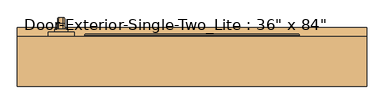
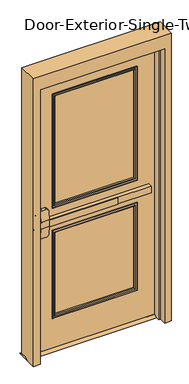
"""IFC4 building model written with IfcOpenShell, lengths in millimetres: door geometry."""

from ifc_helpers import new_model, si_unit, point, frame, frame_2d, origin, place, context, project, spatial, polyline, circle_curve, ellipse_curve, trimmed, segment, composite_curve, outline, extrude, faceted_brep, source, transform, mapped, element, save
from ifc_brep_helpers import plane_surface, cylinder_surface, revolved_surface, advanced_brep


def door_7385851d(model_context):
    return source(origin(), model_context, "Body", "SolidModel", [
        extrude(outline(polyline([(12.7, 12.7), (57.15, 12.7), (82.55, 0.0), (-12.7, 0.0), (12.7, 12.7)])), frame((-508.0, 0.0, 0.0), z_axis=(1.0, 0.0, 0.0), x_axis=(0.0, 1.0, 0.0)), (0.0, 0.0, 1.0), 1016.0),
        extrude(outline(polyline([(150.2833333, -25.4), (-349.25, -25.4), (-349.25, -19.05), (150.2833333, -19.05), (150.2833333, -25.4)])), frame((0.0, 0.0, 990.6), z_axis=(0.0, 0.0, 1.0), x_axis=(1.0, 0.0, 0.0)), (0.0, 0.0, 1.0), 50.8),
        advanced_brep(
        [(-412.75, -19.05, 1041.4), (-412.75, -19.05, 990.6), (-349.25, -19.05, 990.6), (400.05, -19.05, 990.6), (400.05, -19.05, 1041.4), (-349.25, -19.05, 1041.4), (400.05, 12.7, 1041.4), (400.05, 12.7, 990.6), (-349.25, 12.7, 990.6), (-349.25, 12.7, 927.1), (-368.3, 12.7, 908.05), (-393.7, 12.7, 908.05), (-412.75, 12.7, 927.1), (-412.75, 12.7, 1104.9), (-393.7, 12.7, 1123.95), (-368.3, 12.7, 1123.95), (-349.25, 12.7, 1104.9), (-349.25, 12.7, 1041.4), (-349.25, -15.8747533, 1041.4), (-412.75, -15.8747533, 1041.4), (-412.75, -10.8645731, 1104.9), (-412.75, -10.8645731, 927.1), (-412.75, -15.8747533, 990.6), (-349.25, -15.8747533, 990.6), (-349.25, -10.8645731, 927.1), (-349.25, -10.8645731, 1104.9), (-393.7, -9.361519, 1123.95), (-368.3, -9.361519, 1123.95), (-368.3, -9.361519, 908.05), (-393.7, -9.361519, 908.05)],
        [
            (0, 1),
            (1, 2),
            (2, 3),
            (3, 4),
            (4, 5),
            (5, 0),
            (6, 7),
            (7, 8),
            (8, 9),
            (9, 10, circle_curve(frame((-368.3, 12.7, 927.1), z_axis=(0.0, 1.0, 0.0), x_axis=(1.0, 0.0, 0.0)), 19.05)),
            (10, 11),
            (11, 12, circle_curve(frame((-393.7, 12.7, 927.1), z_axis=(0.0, 1.0, 0.0), x_axis=(1.0, 0.0, 0.0)), 19.05)),
            (12, 13),
            (13, 14, circle_curve(frame((-393.7, 12.7, 1104.9), z_axis=(0.0, 1.0, 0.0), x_axis=(1.0, 0.0, 0.0)), 19.05)),
            (14, 15),
            (15, 16, circle_curve(frame((-368.3, 12.7, 1104.9), z_axis=(0.0, 1.0, 0.0), x_axis=(1.0, 0.0, 0.0)), 19.05)),
            (16, 17),
            (17, 6),
            (4, 6),
            (17, 18),
            (18, 19),
            (19, 0),
            (19, 20),
            (20, 13),
            (12, 21),
            (21, 22),
            (22, 1),
            (7, 3),
            (22, 23),
            (23, 8),
            (23, 24),
            (24, 9),
            (16, 25),
            (25, 18),
            (14, 26),
            (26, 27),
            (27, 15),
            (10, 28),
            (28, 29),
            (29, 11),
            (24, 28, ellipse_curve(frame((-368.3, -10.8645731, 927.1), z_axis=(0.0, 0.9969018152893365, 0.07865602756830282), x_axis=(0.0, -0.07865602756830208, 0.9969018152893365)), 19.1092038, 19.05)),
            (27, 25, ellipse_curve(frame((-368.3, -10.8645731, 1104.9), z_axis=(0.0, 0.9969018152893376, -0.07865602756828934), x_axis=(0.0, -0.078656027568288, -0.9969018152893377)), 19.1092038, 19.05)),
            (20, 26, ellipse_curve(frame((-393.7, -10.8645731, 1104.9), z_axis=(0.0, 0.9969018152893376, -0.07865602756828934), x_axis=(0.0, -0.078656027568288, -0.9969018152893377)), 19.1092038, 19.05)),
            (29, 21, ellipse_curve(frame((-393.7, -10.8645731, 927.1), z_axis=(0.0, 0.9969018152893365, 0.07865602756830282), x_axis=(0.0, -0.07865602756830208, 0.9969018152893365)), 19.1092038, 19.05)),
        ],
        [
            plane_surface(frame((-412.75, -19.05, 1041.4), z_axis=(0.0, -1.0, 0.0), x_axis=(-1.0, 0.0, 0.0))),
            plane_surface(frame((-412.75, 12.7, 1041.4), z_axis=(0.0, 1.0, 0.0), x_axis=(1.0, 0.0, 0.0))),
            plane_surface(frame((400.05, -19.05, 1041.4), z_axis=(0.0, 0.0, 1.0), x_axis=(0.0, 1.0, 0.0))),
            plane_surface(frame((-412.75, -19.05, 1041.4), z_axis=(-1.0, 0.0, 0.0), x_axis=(0.0, 1.0, 0.0))),
            plane_surface(frame((-412.75, -19.05, 990.6), z_axis=(0.0, 0.0, -1.0), x_axis=(0.0, 1.0, 0.0))),
            plane_surface(frame((400.05, -19.05, 990.6), z_axis=(1.0, 0.0, 0.0), x_axis=(0.0, 1.0, 0.0))),
            plane_surface(frame((-349.25, -15.8747533, 927.1), z_axis=(1.0, 0.0, 0.0), x_axis=(0.0, 1.0, 0.0))),
            plane_surface(frame((-368.3, -15.8747533, 1123.95), z_axis=(0.0, 0.0, 1.0), x_axis=(0.0, 1.0, 0.0))),
            plane_surface(frame((-393.7, -15.8747533, 908.05), z_axis=(0.0, 0.0, -1.0), x_axis=(0.0, 1.0, 0.0))),
            cylinder_surface(frame((-368.3, 12.7, 927.1), z_axis=(0.0, -1.0, 0.0), x_axis=(1.0, 0.0, 0.0)), 19.05),
            cylinder_surface(frame((-368.3, 12.7, 1104.9), z_axis=(0.0, -1.0, 0.0), x_axis=(1.0, 0.0, 0.0)), 19.05),
            cylinder_surface(frame((-393.7, 12.7, 1104.9), z_axis=(0.0, -1.0, 0.0), x_axis=(1.0, 0.0, 0.0)), 19.05),
            cylinder_surface(frame((-393.7, 12.7, 927.1), z_axis=(0.0, -1.0, 0.0), x_axis=(1.0, 0.0, 0.0)), 19.05),
            plane_surface(frame((-349.25, -15.8747533, 1041.4), z_axis=(0.0, -0.9969018152893376, 0.07865602756828934), x_axis=(-1.0, 0.0, 0.0))),
            plane_surface(frame((-349.25, -9.361519, 908.05), z_axis=(0.0, -0.9969018152893365, -0.07865602756830282), x_axis=(-1.0, 0.0, 0.0))),
        ],
        [
            (0, [[1, 2, 3, 4, 5, 6]]),
            (1, [[7, 8, 9, 10, 11, 12, 13, 14, 15, 16, 17, 18]]),
            (2, [[19, -18, 20, 21, 22, -6, -5]]),
            (3, [[-1, -22, 23, 24, -13, 25, 26, 27]]),
            (4, [[28, -3, -2, -27, 29, 30, -8]]),
            (5, [[-4, -28, -7, -19]]),
            (6, [[-9, -30, 31, 32]]),
            (6, [[-17, 33, 34, -20]]),
            (7, [[-15, 35, 36, 37]]),
            (8, [[-11, 38, 39, 40]]),
            (9, [[-10, -32, 41, -38]]),
            (10, [[-16, -37, 42, -33]]),
            (11, [[-14, -24, 43, -35]]),
            (12, [[-12, -40, 44, -25]]),
            (13, [[-21, -34, -42, -36, -43, -23]]),
            (14, [[-26, -44, -39, -41, -31, -29]]),
        ],
    ),
        advanced_brep(
        [(-391.0, 69.85, 1017.190625), (-391.0, 69.85, 1014.809375), (-387.428125, 69.85, 1011.2375), (-374.5715406, 69.85, 1011.2375), (-371.0, 69.85, 1014.8090406), (-371.0, 69.85, 1017.190625), (-374.571875, 69.85, 1020.7625), (-387.428125, 69.85, 1020.7625), (-391.0, 69.85, 887.809375), (-387.428125, 69.85, 884.2375), (-374.571875, 69.85, 884.2375), (-371.0, 69.85, 887.809375), (-371.0, 69.85, 890.1909594), (-374.5715406, 69.85, 893.7625), (-387.428125, 69.85, 893.7625), (-391.0, 69.85, 890.190625), (-391.0, 95.25, 1017.190625), (-391.0, 109.140625, 1003.3), (-391.0, 109.140625, 901.7), (-391.0, 95.25, 887.809375), (-391.0, 95.25, 890.190625), (-391.0, 106.759375, 901.7), (-391.0, 106.759375, 1003.3), (-391.0, 95.25, 1014.809375), (-387.428125, 95.25, 1011.2375), (-374.5715406, 95.25, 1011.2375), (-371.0, 95.25, 1014.8090406), (-371.0, 106.7590406, 1003.3), (-371.0, 106.7590406, 901.7), (-371.0, 95.25, 890.1909594), (-371.0, 95.25, 887.809375), (-371.0, 109.140625, 901.7), (-371.0, 109.140625, 1003.3), (-371.0, 95.25, 1017.190625), (-374.571875, 95.25, 1020.7625), (-387.428125, 95.25, 1020.7625), (-387.428125, 103.1875, 1003.3), (-374.5715406, 103.1875, 1003.3), (-374.571875, 112.7125, 1003.3), (-387.428125, 112.7125, 1003.3), (-387.428125, 103.1875, 901.7), (-374.5715406, 103.1875, 901.7), (-374.571875, 112.7125, 901.7), (-387.428125, 112.7125, 901.7), (-387.428125, 95.25, 893.7625), (-374.5715406, 95.25, 893.7625), (-374.571875, 95.25, 884.2375), (-387.428125, 95.25, 884.2375)],
        [
            (0, 1),
            (1, 2, circle_curve(frame((-387.428125, 69.85, 1014.809375), z_axis=(0.0, -1.0, 0.0), x_axis=(0.0, 0.0, 1.0)), 3.571875)),
            (2, 3),
            (3, 4, circle_curve(frame((-374.5715406, 69.85, 1014.8090406), z_axis=(0.0, -1.0, 0.0), x_axis=(0.0, 0.0, 1.0)), 3.5715406)),
            (4, 5),
            (5, 6, circle_curve(frame((-374.571875, 69.85, 1017.190625), z_axis=(0.0, -1.0, 0.0), x_axis=(0.0, 0.0, 1.0)), 3.571875)),
            (6, 7),
            (7, 0, circle_curve(frame((-387.428125, 69.85, 1017.190625), z_axis=(0.0, -1.0, 0.0), x_axis=(0.0, 0.0, 1.0)), 3.571875)),
            (8, 9, circle_curve(frame((-387.428125, 69.85, 887.809375), z_axis=(0.0, -1.0, 0.0), x_axis=(0.0, 0.0, -1.0)), 3.571875)),
            (9, 10),
            (10, 11, circle_curve(frame((-374.571875, 69.85, 887.809375), z_axis=(0.0, -1.0, 0.0), x_axis=(0.0, 0.0, -1.0)), 3.571875)),
            (11, 12),
            (12, 13, circle_curve(frame((-374.5715406, 69.85, 890.1909594), z_axis=(0.0, -1.0, 0.0), x_axis=(0.0, 0.0, -1.0)), 3.5715406)),
            (13, 14),
            (14, 15, circle_curve(frame((-387.428125, 69.85, 890.190625), z_axis=(0.0, -1.0, 0.0), x_axis=(0.0, 0.0, -1.0)), 3.571875)),
            (15, 8),
            (0, 16),
            (16, 17, circle_curve(frame((-391.0, 95.25, 1003.3), z_axis=(-1.0, 0.0, 0.0), x_axis=(0.0, 0.0, 1.0)), 13.890625)),
            (17, 18),
            (18, 19, circle_curve(frame((-391.0, 95.25, 901.7), z_axis=(-1.0, 0.0, 0.0), x_axis=(0.0, 1.0, 0.0)), 13.890625)),
            (19, 8),
            (15, 20),
            (20, 21, circle_curve(frame((-391.0, 95.25, 901.7), z_axis=(1.0, 0.0, 0.0), x_axis=(0.0, 1.0, 0.0)), 11.509375)),
            (21, 22),
            (22, 23, circle_curve(frame((-391.0, 95.25, 1003.3), z_axis=(1.0, 0.0, 0.0), x_axis=(0.0, 0.0, 1.0)), 11.509375)),
            (23, 1),
            (23, 24, circle_curve(frame((-387.428125, 95.25, 1014.809375), z_axis=(0.0, -1.0, 0.0), x_axis=(0.0, 0.0, 1.0)), 3.571875)),
            (24, 2),
            (24, 25),
            (25, 3),
            (25, 26, circle_curve(frame((-374.5715406, 95.25, 1014.8090406), z_axis=(0.0, -1.0, 0.0), x_axis=(0.0, 0.0, 1.0)), 3.5715406)),
            (26, 4),
            (26, 27, circle_curve(frame((-371.0, 95.25, 1003.3), z_axis=(-1.0, 0.0, 0.0), x_axis=(0.0, 0.0, 1.0)), 11.5090406)),
            (27, 28),
            (28, 29, circle_curve(frame((-371.0, 95.25, 901.7), z_axis=(-1.0, 0.0, 0.0), x_axis=(0.0, 1.0, 0.0)), 11.5090406)),
            (29, 12),
            (11, 30),
            (30, 31, circle_curve(frame((-371.0, 95.25, 901.7), z_axis=(1.0, 0.0, 0.0), x_axis=(0.0, 1.0, 0.0)), 13.890625)),
            (31, 32),
            (32, 33, circle_curve(frame((-371.0, 95.25, 1003.3), z_axis=(1.0, 0.0, 0.0), x_axis=(0.0, 0.0, 1.0)), 13.890625)),
            (33, 5),
            (33, 34, circle_curve(frame((-374.571875, 95.25, 1017.190625), z_axis=(0.0, -1.0, 0.0), x_axis=(0.0, 0.0, 1.0)), 3.571875)),
            (34, 6),
            (34, 35),
            (35, 7),
            (35, 16, circle_curve(frame((-387.428125, 95.25, 1017.190625), z_axis=(0.0, -1.0, 0.0), x_axis=(0.0, 0.0, 1.0)), 3.571875)),
            (36, 24, circle_curve(frame((-387.428125, 95.25, 1003.3), z_axis=(1.0, 0.0, 0.0), x_axis=(0.0, 0.0, 1.0)), 7.9375)),
            (22, 36, circle_curve(frame((-387.428125, 106.759375, 1003.3), z_axis=(0.0, 0.0, 1.0), x_axis=(0.0, 1.0, 0.0)), 3.571875)),
            (37, 25, circle_curve(frame((-374.5715406, 95.25, 1003.3), z_axis=(1.0, 0.0, 0.0), x_axis=(0.0, 0.0, 1.0)), 7.9375)),
            (36, 37),
            (37, 27, circle_curve(frame((-374.5715406, 106.7590406, 1003.3), z_axis=(0.0, 0.0, 1.0), x_axis=(0.0, 1.0, 0.0)), 3.5715406)),
            (38, 34, circle_curve(frame((-374.571875, 95.25, 1003.3), z_axis=(1.0, 0.0, 0.0), x_axis=(0.0, 0.0, 1.0)), 17.4625)),
            (32, 38, circle_curve(frame((-374.571875, 109.140625, 1003.3), z_axis=(0.0, 0.0, 1.0), x_axis=(0.0, 1.0, 0.0)), 3.571875)),
            (39, 35, circle_curve(frame((-387.428125, 95.25, 1003.3), z_axis=(1.0, 0.0, 0.0), x_axis=(0.0, 0.0, 1.0)), 17.4625)),
            (38, 39),
            (39, 17, circle_curve(frame((-387.428125, 109.140625, 1003.3), z_axis=(0.0, 0.0, 1.0), x_axis=(0.0, 1.0, 0.0)), 3.571875)),
            (21, 40, circle_curve(frame((-387.428125, 106.759375, 901.7), z_axis=(0.0, 0.0, 1.0), x_axis=(0.0, 1.0, 0.0)), 3.571875)),
            (40, 36),
            (40, 41),
            (41, 37),
            (41, 28, circle_curve(frame((-374.5715406, 106.7590406, 901.7), z_axis=(0.0, 0.0, 1.0), x_axis=(0.0, 1.0, 0.0)), 3.5715406)),
            (31, 42, circle_curve(frame((-374.571875, 109.140625, 901.7), z_axis=(0.0, 0.0, 1.0), x_axis=(0.0, 1.0, 0.0)), 3.571875)),
            (42, 38),
            (42, 43),
            (43, 39),
            (43, 18, circle_curve(frame((-387.428125, 109.140625, 901.7), z_axis=(0.0, 0.0, 1.0), x_axis=(0.0, 1.0, 0.0)), 3.571875)),
            (44, 40, circle_curve(frame((-387.428125, 95.25, 901.7), z_axis=(1.0, 0.0, 0.0), x_axis=(0.0, 1.0, 0.0)), 7.9375)),
            (20, 44, circle_curve(frame((-387.428125, 95.25, 890.190625), z_axis=(0.0, 1.0, 0.0), x_axis=(0.0, 0.0, -1.0)), 3.571875)),
            (45, 41, circle_curve(frame((-374.5715406, 95.25, 901.7), z_axis=(1.0, 0.0, 0.0), x_axis=(0.0, 1.0, 0.0)), 7.9375)),
            (44, 45),
            (45, 29, circle_curve(frame((-374.5715406, 95.25, 890.1909594), z_axis=(0.0, 1.0, 0.0), x_axis=(0.0, 0.0, -1.0)), 3.5715406)),
            (46, 42, circle_curve(frame((-374.571875, 95.25, 901.7), z_axis=(1.0, 0.0, 0.0), x_axis=(0.0, 1.0, 0.0)), 17.4625)),
            (30, 46, circle_curve(frame((-374.571875, 95.25, 887.809375), z_axis=(0.0, 1.0, 0.0), x_axis=(0.0, 0.0, -1.0)), 3.571875)),
            (47, 43, circle_curve(frame((-387.428125, 95.25, 901.7), z_axis=(1.0, 0.0, 0.0), x_axis=(0.0, 1.0, 0.0)), 17.4625)),
            (46, 47),
            (47, 19, circle_curve(frame((-387.428125, 95.25, 887.809375), z_axis=(0.0, 1.0, 0.0), x_axis=(0.0, 0.0, -1.0)), 3.571875)),
            (14, 44),
            (13, 45),
            (10, 46),
            (9, 47),
        ],
        [
            plane_surface(frame((-381.0, 69.85, 1016.0), z_axis=(0.0, -1.0, 0.0), x_axis=(1.0, 0.0, 0.0))),
            plane_surface(frame((-381.0, 69.85, 889.0), z_axis=(0.0, -1.0, 0.0), x_axis=(1.0, 0.0, 0.0))),
            plane_surface(frame((-391.0, 69.85, 1017.190625), z_axis=(-1.0, 0.0, 0.0), x_axis=(0.0, 1.0, 0.0))),
            cylinder_surface(frame((-387.428125, 69.85, 1014.809375), z_axis=(0.0, -1.0, 0.0), x_axis=(0.0, 0.0, 1.0)), 3.571875),
            plane_surface(frame((-387.428125, 69.85, 1011.2375), z_axis=(0.0, 0.0, -1.0), x_axis=(0.0, 1.0, 0.0))),
            cylinder_surface(frame((-374.5715406, 69.85, 1014.8090406), z_axis=(0.0, -1.0, 0.0), x_axis=(0.0, 0.0, 1.0)), 3.5715406),
            plane_surface(frame((-371.0, 69.85, 1014.8090406), z_axis=(1.0, 0.0, 0.0), x_axis=(0.0, 1.0, 0.0))),
            cylinder_surface(frame((-374.571875, 69.85, 1017.190625), z_axis=(0.0, -1.0, 0.0), x_axis=(0.0, 0.0, 1.0)), 3.571875),
            plane_surface(frame((-374.571875, 69.85, 1020.7625), z_axis=(0.0, 0.0, 1.0), x_axis=(0.0, 1.0, 0.0))),
            cylinder_surface(frame((-387.428125, 69.85, 1017.190625), z_axis=(0.0, -1.0, 0.0), x_axis=(0.0, 0.0, 1.0)), 3.571875),
            revolved_surface(trimmed(ellipse_curve(frame((-387.428125, 95.25, 1014.809375), z_axis=(0.0, -1.0, 0.0), x_axis=(0.0, 0.0, 1.0)), 3.571875, 3.571875), [point((-391.0, 95.25, 1014.809375))], [point((-387.428125, 95.25, 1011.2375))], True, "CARTESIAN"), (-381.0, 95.25, 1003.3), (-1.0, 0.0, 0.0)),
            revolved_surface(polyline([(-387.428125, 95.25, 1011.2375), (-374.5715406, 95.25, 1011.2375)]), (-381.0, 95.25, 1003.3), (-1.0, 0.0, 0.0)),
            revolved_surface(trimmed(ellipse_curve(frame((-374.5715406, 95.25, 1014.8090406), z_axis=(0.0, -1.0, 0.0), x_axis=(0.0, 0.0, 1.0)), 3.5715406, 3.5715406), [point((-374.5715406, 95.25, 1011.2375))], [point((-371.0, 95.25, 1014.8090406))], True, "CARTESIAN"), (-381.0, 95.25, 1003.3), (-1.0, 0.0, 0.0)),
            revolved_surface(trimmed(ellipse_curve(frame((-374.571875, 95.25, 1017.190625), z_axis=(0.0, -1.0, 0.0), x_axis=(0.0, 0.0, 1.0)), 3.571875, 3.571875), [point((-371.0, 95.25, 1017.190625))], [point((-374.571875, 95.25, 1020.7625))], True, "CARTESIAN"), (-381.0, 95.25, 1003.3), (-1.0, 0.0, 0.0)),
            cylinder_surface(frame((-381.0, 95.25, 1003.3), z_axis=(-1.0, 0.0, 0.0), x_axis=(0.0, 0.0, 1.0)), 17.4625),
            revolved_surface(trimmed(ellipse_curve(frame((-387.428125, 95.25, 1017.190625), z_axis=(0.0, -1.0, 0.0), x_axis=(0.0, 0.0, 1.0)), 3.571875, 3.571875), [point((-387.428125, 95.25, 1020.7625))], [point((-391.0, 95.25, 1017.190625))], True, "CARTESIAN"), (-381.0, 95.25, 1003.3), (-1.0, 0.0, 0.0)),
            cylinder_surface(frame((-387.428125, 106.759375, 1003.3), z_axis=(0.0, 0.0, 1.0), x_axis=(0.0, 1.0, 0.0)), 3.571875),
            plane_surface(frame((-387.428125, 103.1875, 1003.3), z_axis=(0.0, -1.0, 0.0), x_axis=(0.0, 0.0, -1.0))),
            cylinder_surface(frame((-374.5715406, 106.7590406, 1003.3), z_axis=(0.0, 0.0, 1.0), x_axis=(0.0, 1.0, 0.0)), 3.5715406),
            cylinder_surface(frame((-374.571875, 109.140625, 1003.3), z_axis=(0.0, 0.0, 1.0), x_axis=(0.0, 1.0, 0.0)), 3.571875),
            plane_surface(frame((-374.571875, 112.7125, 1003.3), z_axis=(0.0, 1.0, 0.0), x_axis=(0.0, 0.0, -1.0))),
            cylinder_surface(frame((-387.428125, 109.140625, 1003.3), z_axis=(0.0, 0.0, 1.0), x_axis=(0.0, 1.0, 0.0)), 3.571875),
            revolved_surface(trimmed(ellipse_curve(frame((-387.428125, 106.759375, 901.7), z_axis=(0.0, 0.0, 1.0), x_axis=(0.0, 1.0, 0.0)), 3.571875, 3.571875), [point((-391.0, 106.759375, 901.7))], [point((-387.428125, 103.1875, 901.7))], True, "CARTESIAN"), (-381.0, 95.25, 901.7), (-1.0, 0.0, 0.0)),
            revolved_surface(polyline([(-387.428125, 103.1875, 901.7), (-374.5715406, 103.1875, 901.7)]), (-381.0, 95.25, 901.7), (-1.0, 0.0, 0.0)),
            revolved_surface(trimmed(ellipse_curve(frame((-374.5715406, 106.7590406, 901.7), z_axis=(0.0, 0.0, 1.0), x_axis=(0.0, 1.0, 0.0)), 3.5715406, 3.5715406), [point((-374.5715406, 103.1875, 901.7))], [point((-371.0, 106.7590406, 901.7))], True, "CARTESIAN"), (-381.0, 95.25, 901.7), (-1.0, 0.0, 0.0)),
            revolved_surface(trimmed(ellipse_curve(frame((-374.571875, 109.140625, 901.7), z_axis=(0.0, 0.0, 1.0), x_axis=(0.0, 1.0, 0.0)), 3.571875, 3.571875), [point((-371.0, 109.140625, 901.7))], [point((-374.571875, 112.7125, 901.7))], True, "CARTESIAN"), (-381.0, 95.25, 901.7), (-1.0, 0.0, 0.0)),
            cylinder_surface(frame((-381.0, 95.25, 901.7), z_axis=(-1.0, 0.0, 0.0), x_axis=(0.0, 1.0, 0.0)), 17.4625),
            revolved_surface(trimmed(ellipse_curve(frame((-387.428125, 109.140625, 901.7), z_axis=(0.0, 0.0, 1.0), x_axis=(0.0, 1.0, 0.0)), 3.571875, 3.571875), [point((-387.428125, 112.7125, 901.7))], [point((-391.0, 109.140625, 901.7))], True, "CARTESIAN"), (-381.0, 95.25, 901.7), (-1.0, 0.0, 0.0)),
            cylinder_surface(frame((-387.428125, 95.25, 890.190625), z_axis=(0.0, 1.0, 0.0), x_axis=(0.0, 0.0, -1.0)), 3.571875),
            plane_surface(frame((-387.428125, 95.25, 893.7625), z_axis=(0.0, 0.0, 1.0), x_axis=(0.0, -1.0, 0.0))),
            cylinder_surface(frame((-374.5715406, 95.25, 890.1909594), z_axis=(0.0, 1.0, 0.0), x_axis=(0.0, 0.0, -1.0)), 3.5715406),
            cylinder_surface(frame((-374.571875, 95.25, 887.809375), z_axis=(0.0, 1.0, 0.0), x_axis=(0.0, 0.0, -1.0)), 3.571875),
            plane_surface(frame((-374.571875, 95.25, 884.2375), z_axis=(0.0, 0.0, -1.0), x_axis=(0.0, -1.0, 0.0))),
            cylinder_surface(frame((-387.428125, 95.25, 887.809375), z_axis=(0.0, 1.0, 0.0), x_axis=(0.0, 0.0, -1.0)), 3.571875),
        ],
        [
            (0, [[1, 2, 3, 4, 5, 6, 7, 8]]),
            (1, [[9, 10, 11, 12, 13, 14, 15, 16]]),
            (2, [[-1, 17, 18, 19, 20, 21, -16, 22, 23, 24, 25, 26]]),
            (3, [[-2, -26, 27, 28]]),
            (4, [[-3, -28, 29, 30]]),
            (5, [[-4, -30, 31, 32]]),
            (6, [[-5, -32, 33, 34, 35, 36, -12, 37, 38, 39, 40, 41]]),
            (7, [[-6, -41, 42, 43]]),
            (8, [[-7, -43, 44, 45]]),
            (9, [[-8, -45, 46, -17]]),
            (10, [[47, -27, -25, 48]]),
            (11, [[49, -29, -47, 50]]),
            (12, [[-33, -31, -49, 51]]),
            (13, [[52, -42, -40, 53]]),
            (14, [[54, -44, -52, 55]]),
            (15, [[-18, -46, -54, 56]]),
            (16, [[-48, -24, 57, 58]]),
            (17, [[-50, -58, 59, 60]]),
            (18, [[-51, -60, 61, -34]]),
            (19, [[-53, -39, 62, 63]]),
            (20, [[-55, -63, 64, 65]]),
            (21, [[-56, -65, 66, -19]]),
            (22, [[67, -57, -23, 68]]),
            (23, [[69, -59, -67, 70]]),
            (24, [[-35, -61, -69, 71]]),
            (25, [[72, -62, -38, 73]]),
            (26, [[74, -64, -72, 75]]),
            (27, [[-20, -66, -74, 76]]),
            (28, [[-68, -22, -15, 77]]),
            (29, [[-70, -77, -14, 78]]),
            (30, [[-71, -78, -13, -36]]),
            (31, [[-73, -37, -11, 79]]),
            (32, [[-75, -79, -10, 80]]),
            (33, [[-76, -80, -9, -21]]),
        ],
    ),
        extrude(outline(composite_curve([segment(trimmed(circle_curve(frame_2d((1117.6, -381.0)), 19.0), [point((1117.6, -400.0))], [point((1117.6, -362.0))], False, "CARTESIAN"), True, "CONTINUOUS"), segment(trimmed(circle_curve(frame_2d((1117.6, -381.0)), 19.0), [point((1117.6, -362.0))], [point((1117.6, -400.0))], False, "CARTESIAN"), True, "CONTINUOUS")], self_intersect=False)), frame((0.0, 69.85, 0.0), z_axis=(0.0, 1.0, 0.0), x_axis=(0.0, 0.0, 1.0)), (0.0, 0.0, 1.0), 8.73125),
        extrude(outline(composite_curve([segment(trimmed(circle_curve(frame_2d((1113.0338574, -381.0)), 89.3016225), [point((1193.8, -342.9))], [point((1193.8, -419.1))], False, "CARTESIAN"), True, "CONTINUOUS"), segment(polyline([(1193.8, -419.1), (838.2, -419.1)]), True, "CONTINUOUS"), segment(trimmed(circle_curve(frame_2d((918.9661426, -381.0)), 89.3016225), [point((838.2, -419.1))], [point((838.2, -342.9))], False, "CARTESIAN"), True, "CONTINUOUS"), segment(polyline([(838.2, -342.9), (1193.8, -342.9)]), True, "CONTINUOUS")], self_intersect=False)), frame((0.0, 57.15, 0.0), z_axis=(0.0, 1.0, 0.0), x_axis=(0.0, 0.0, 1.0)), (0.0, 0.0, 1.0), 12.7),
        faceted_brep([(457.2, 7.9375, 0.0), (457.2, 57.15, 0.0), (508.0, 57.15, 0.0), (508.0, -88.9, 0.0), (457.2, -88.9, 0.0), (457.2, -39.6875, 0.0), (441.325, -39.6875, 0.0), (441.325, 7.9375, 0.0), (457.2, 7.9375, 2133.6), (457.2, 57.15, 2133.6), (-457.2, 57.15, 2133.6), (-457.2, 57.15, 0.0), (-508.0, 57.15, 0.0), (-508.0, 57.15, 2235.2), (508.0, 57.15, 2235.2), (508.0, -88.9, 2235.2), (-508.0, -88.9, 2235.2), (-508.0, -88.9, 0.0), (-457.2, -88.9, 0.0), (-457.2, -88.9, 2133.6), (457.2, -88.9, 2133.6), (457.2, -39.6875, 2133.6), (-457.2, -39.6875, 2133.6), (-457.2, -39.6875, 0.0), (-441.325, -39.6875, 0.0), (-441.325, -39.6875, 2117.725), (441.325, -39.6875, 2117.725), (441.325, 7.9375, 2117.725), (-441.325, 7.9375, 2117.725), (-441.325, 7.9375, 0.0), (-457.2, 7.9375, 0.0), (-457.2, 7.9375, 2133.6)], [[[0, 1, 2, 3, 4, 5, 6, 7]], [[1, 0, 8, 9]], [[2, 1, 9, 10, 11, 12, 13, 14]], [[3, 2, 14, 15]], [[4, 3, 15, 16, 17, 18, 19, 20]], [[5, 4, 20, 21]], [[6, 5, 21, 22, 23, 24, 25, 26]], [[7, 6, 26, 27]], [[0, 7, 27, 28, 29, 30, 31, 8]], [[9, 8, 31, 10]], [[20, 19, 22, 21]], [[26, 25, 28, 27]], [[12, 11, 30, 29, 24, 23, 18, 17]], [[11, 10, 31, 30]], [[13, 12, 17, 16]], [[19, 18, 23, 22]], [[25, 24, 29, 28]], [[15, 14, 13, 16]]]),
        extrude(outline(polyline([(2133.6, -457.2), (12.7, -457.2), (12.7, 457.2), (2133.6, 457.2), (2133.6, -457.2)]), holes=[polyline([(1981.2, -304.8), (1981.2, 304.8), (1111.25, 304.8), (1111.25, -304.8), (1981.2, -304.8)]), polyline([(920.75, -304.8), (920.75, 304.8), (254.0, 304.8), (254.0, -304.8), (920.75, -304.8)])]), frame((0.0, 12.7, 0.0), z_axis=(0.0, 1.0, 0.0), x_axis=(0.0, 0.0, 1.0)), (0.0, 0.0, 1.0), 44.45),
        extrude(outline(polyline([(304.8, 25.4), (-304.8, 25.4), (-304.8, 44.45), (304.8, 44.45), (304.8, 25.4)])), frame((0.0, 0.0, 1111.25), z_axis=(0.0, 0.0, 1.0), x_axis=(1.0, 0.0, 0.0)), (0.0, 0.0, 1.0), 869.95),
        extrude(outline(polyline([(304.8, 25.4), (-304.8, 25.4), (-304.8, 44.45), (304.8, 44.45), (304.8, 25.4)])), frame((0.0, 0.0, 254.0), z_axis=(0.0, 0.0, 1.0), x_axis=(1.0, 0.0, 0.0)), (0.0, 0.0, 1.0), 666.75),
        advanced_brep(
        [(304.8, 25.4, 920.75), (304.8, 12.7, 920.75), (304.8, 12.7, 254.0), (304.8, 25.4, 254.0), (292.8, 11.7, 908.75), (292.8, 25.4, 908.75), (292.8, 25.4, 266.0), (292.8, 11.7, 266.0), (297.8, 6.7, 913.75), (297.8, 6.7, 261.0), (312.8, 8.7, 928.75), (310.8, 6.7, 926.75), (310.8, 6.7, 248.0), (312.8, 8.7, 246.0), (312.8, 12.7, 928.75), (312.8, 12.7, 246.0), (-304.8, 12.7, 254.0), (-304.8, 25.4, 254.0), (-292.8, 25.4, 266.0), (-292.8, 11.7, 266.0), (-297.8, 6.7, 261.0), (-310.8, 6.7, 248.0), (-312.8, 8.7, 246.0), (-312.8, 12.7, 246.0), (-304.8, 12.7, 920.75), (-304.8, 25.4, 920.75), (-292.8, 25.4, 908.75), (-292.8, 11.7, 908.75), (-297.8, 6.7, 913.75), (-310.8, 6.7, 926.75), (-312.8, 8.7, 928.75), (-312.8, 12.7, 928.75)],
        [
            (0, 1),
            (1, 2),
            (2, 3),
            (3, 0),
            (4, 5),
            (5, 6),
            (6, 7),
            (7, 4),
            (8, 4, ellipse_curve(frame((297.8, 11.7, 913.75), z_axis=(0.7071067811865475, 0.0, -0.7071067811865475), x_axis=(0.7071067811865474, 0.0, 0.7071067811865476)), 7.0710678, 5.0)),
            (7, 9, ellipse_curve(frame((297.8, 11.7, 261.0), z_axis=(0.7071067811865475, 0.0, 0.7071067811865475), x_axis=(-0.7071067811865474, 0.0, 0.7071067811865476)), 7.0710678, 5.0)),
            (9, 8),
            (10, 11, ellipse_curve(frame((310.8, 8.7, 926.75), z_axis=(0.7071067811865475, 0.0, -0.7071067811865475), x_axis=(0.7071067811865474, 0.0, 0.7071067811865476)), 2.8284271, 2.0)),
            (11, 12),
            (12, 13, ellipse_curve(frame((310.8, 8.7, 248.0), z_axis=(0.7071067811865475, 0.0, 0.7071067811865475), x_axis=(-0.7071067811865474, 0.0, 0.7071067811865476)), 2.8284271, 2.0)),
            (13, 10),
            (14, 10),
            (13, 15),
            (15, 14),
            (2, 16),
            (16, 17),
            (17, 3),
            (6, 18),
            (18, 19),
            (19, 7),
            (19, 20, ellipse_curve(frame((-297.8, 11.7, 261.0), z_axis=(0.7071067811865475, 0.0, -0.7071067811865475), x_axis=(0.7071067811865476, 0.0, 0.7071067811865474)), 7.0710678, 5.0)),
            (20, 9),
            (12, 21),
            (21, 22, ellipse_curve(frame((-310.8, 8.7, 248.0), z_axis=(0.7071067811865475, 0.0, -0.7071067811865475), x_axis=(0.7071067811865476, 0.0, 0.7071067811865474)), 2.8284271, 2.0)),
            (22, 13),
            (22, 23),
            (23, 15),
            (16, 24),
            (24, 25),
            (25, 17),
            (18, 26),
            (26, 27),
            (27, 19),
            (27, 28, ellipse_curve(frame((-297.8, 11.7, 913.75), z_axis=(-0.7071067811865475, 0.0, -0.7071067811865475), x_axis=(0.7071067811865474, 0.0, -0.7071067811865476)), 7.0710678, 5.0)),
            (28, 20),
            (21, 29),
            (29, 30, ellipse_curve(frame((-310.8, 8.7, 926.75), z_axis=(-0.7071067811865475, 0.0, -0.7071067811865475), x_axis=(0.7071067811865474, 0.0, -0.7071067811865476)), 2.8284271, 2.0)),
            (30, 22),
            (30, 31),
            (31, 23),
            (31, 14),
            (1, 24),
            (0, 25),
            (5, 26),
            (4, 27),
            (8, 28),
            (11, 29),
            (10, 30),
        ],
        [
            plane_surface(frame((304.8, 12.7, 920.75), z_axis=(1.0, 0.0, 0.0), x_axis=(0.0, 0.0, -1.0))),
            plane_surface(frame((292.8, 25.4, 908.75), z_axis=(-1.0, 0.0, 0.0), x_axis=(0.0, 0.0, -1.0))),
            cylinder_surface(frame((297.8, 11.7, 920.75), z_axis=(0.0, 0.0, 1.0), x_axis=(1.0, 0.0, 0.0)), 5.0),
            cylinder_surface(frame((310.8, 8.7, 920.75), z_axis=(0.0, 0.0, 1.0), x_axis=(1.0, 0.0, 0.0)), 2.0),
            plane_surface(frame((312.8, 8.7, 928.75), z_axis=(1.0, 0.0, 0.0), x_axis=(0.0, 0.0, -1.0))),
            plane_surface(frame((304.8, 12.7, 254.0), z_axis=(0.0, 0.0, -1.0), x_axis=(-1.0, 0.0, 0.0))),
            plane_surface(frame((292.8, 25.4, 266.0), z_axis=(0.0, 0.0, 1.0), x_axis=(-1.0, 0.0, 0.0))),
            cylinder_surface(frame((304.8, 11.7, 261.0), z_axis=(1.0, 0.0, 0.0), x_axis=(0.0, 0.0, -1.0)), 5.0),
            cylinder_surface(frame((304.8, 8.7, 248.0), z_axis=(1.0, 0.0, 0.0), x_axis=(0.0, 0.0, -1.0)), 2.0),
            plane_surface(frame((312.8, 8.7, 246.0), z_axis=(0.0, 0.0, -1.0), x_axis=(-1.0, 0.0, 0.0))),
            plane_surface(frame((-304.8, 12.7, 254.0), z_axis=(-1.0, 0.0, 0.0), x_axis=(0.0, 0.0, 1.0))),
            plane_surface(frame((-292.8, 25.4, 266.0), z_axis=(1.0, 0.0, 0.0), x_axis=(0.0, 0.0, 1.0))),
            cylinder_surface(frame((-297.8, 11.7, 254.0), z_axis=(0.0, 0.0, -1.0), x_axis=(-1.0, 0.0, 0.0)), 5.0),
            cylinder_surface(frame((-310.8, 8.7, 254.0), z_axis=(0.0, 0.0, -1.0), x_axis=(-1.0, 0.0, 0.0)), 2.0),
            plane_surface(frame((-312.8, 8.7, 246.0), z_axis=(-1.0, 0.0, 0.0), x_axis=(0.0, 0.0, 1.0))),
            plane_surface(frame((-312.8, 12.7, 928.75), z_axis=(0.0, 1.0, 0.0), x_axis=(1.0, 0.0, 0.0))),
            plane_surface(frame((-304.8, 12.7, 920.75), z_axis=(0.0, 0.0, 1.0), x_axis=(1.0, 0.0, 0.0))),
            plane_surface(frame((-304.8, 25.4, 920.75), z_axis=(0.0, 1.0, 0.0), x_axis=(1.0, 0.0, 0.0))),
            plane_surface(frame((-292.8, 25.4, 908.75), z_axis=(0.0, 0.0, -1.0), x_axis=(1.0, 0.0, 0.0))),
            cylinder_surface(frame((-304.8, 11.7, 913.75), z_axis=(-1.0, 0.0, 0.0), x_axis=(0.0, 0.0, 1.0)), 5.0),
            plane_surface(frame((-297.8, 6.7, 913.75), z_axis=(0.0, -1.0, 0.0), x_axis=(1.0, 0.0, 0.0))),
            cylinder_surface(frame((-304.8, 8.7, 926.75), z_axis=(-1.0, 0.0, 0.0), x_axis=(0.0, 0.0, 1.0)), 2.0),
            plane_surface(frame((-312.8, 8.7, 928.75), z_axis=(0.0, 0.0, 1.0), x_axis=(1.0, 0.0, 0.0))),
        ],
        [
            (0, [[1, 2, 3, 4]]),
            (1, [[5, 6, 7, 8]]),
            (2, [[9, -8, 10, 11]]),
            (3, [[12, 13, 14, 15]]),
            (4, [[16, -15, 17, 18]]),
            (5, [[-3, 19, 20, 21]]),
            (6, [[-7, 22, 23, 24]]),
            (7, [[-10, -24, 25, 26]]),
            (8, [[-14, 27, 28, 29]]),
            (9, [[-17, -29, 30, 31]]),
            (10, [[-20, 32, 33, 34]]),
            (11, [[-23, 35, 36, 37]]),
            (12, [[-25, -37, 38, 39]]),
            (13, [[-28, 40, 41, 42]]),
            (14, [[-30, -42, 43, 44]]),
            (15, [[-31, -44, 45, -18], [46, -32, -19, -2]]),
            (16, [[-33, -46, -1, 47]]),
            (17, [[-21, -34, -47, -4], [48, -35, -22, -6]]),
            (18, [[-36, -48, -5, 49]]),
            (19, [[-38, -49, -9, 50]]),
            (20, [[51, -40, -27, -13], [-26, -39, -50, -11]]),
            (21, [[-41, -51, -12, 52]]),
            (22, [[-43, -52, -16, -45]]),
        ],
    ),
        advanced_brep(
        [(-304.8, 44.45, 920.75), (-304.8, 57.15, 920.75), (-304.8, 57.15, 254.0), (-304.8, 44.45, 254.0), (-292.8, 58.15, 908.75), (-292.8, 44.45, 908.75), (-292.8, 44.45, 266.0), (-292.8, 58.15, 266.0), (-297.8, 63.15, 913.75), (-297.8, 63.15, 261.0), (-312.8, 61.15, 928.75), (-310.8, 63.15, 926.75), (-310.8, 63.15, 248.0), (-312.8, 61.15, 246.0), (-312.8, 57.15, 928.75), (-312.8, 57.15, 246.0), (304.8, 57.15, 254.0), (304.8, 44.45, 254.0), (292.8, 44.45, 266.0), (292.8, 58.15, 266.0), (297.8, 63.15, 261.0), (310.8, 63.15, 248.0), (312.8, 61.15, 246.0), (312.8, 57.15, 246.0), (304.8, 57.15, 920.75), (304.8, 44.45, 920.75), (292.8, 44.45, 908.75), (292.8, 58.15, 908.75), (297.8, 63.15, 913.75), (310.8, 63.15, 926.75), (312.8, 61.15, 928.75), (312.8, 57.15, 928.75)],
        [
            (0, 1),
            (1, 2),
            (2, 3),
            (3, 0),
            (4, 5),
            (5, 6),
            (6, 7),
            (7, 4),
            (8, 4, ellipse_curve(frame((-297.8, 58.15, 913.75), z_axis=(-0.7071067811865475, 0.0, -0.7071067811865475), x_axis=(-0.7071067811865474, 0.0, 0.7071067811865476)), 7.0710678, 5.0)),
            (7, 9, ellipse_curve(frame((-297.8, 58.15, 261.0), z_axis=(-0.7071067811865475, 0.0, 0.7071067811865475), x_axis=(0.7071067811865474, 0.0, 0.7071067811865476)), 7.0710678, 5.0)),
            (9, 8),
            (10, 11, ellipse_curve(frame((-310.8, 61.15, 926.75), z_axis=(-0.7071067811865475, 0.0, -0.7071067811865475), x_axis=(-0.7071067811865474, 0.0, 0.7071067811865476)), 2.8284271, 2.0)),
            (11, 12),
            (12, 13, ellipse_curve(frame((-310.8, 61.15, 248.0), z_axis=(-0.7071067811865475, 0.0, 0.7071067811865475), x_axis=(0.7071067811865474, 0.0, 0.7071067811865476)), 2.8284271, 2.0)),
            (13, 10),
            (14, 10),
            (13, 15),
            (15, 14),
            (2, 16),
            (16, 17),
            (17, 3),
            (6, 18),
            (18, 19),
            (19, 7),
            (19, 20, ellipse_curve(frame((297.8, 58.15, 261.0), z_axis=(-0.7071067811865475, 0.0, -0.7071067811865475), x_axis=(-0.7071067811865476, 0.0, 0.7071067811865474)), 7.0710678, 5.0)),
            (20, 9),
            (12, 21),
            (21, 22, ellipse_curve(frame((310.8, 61.15, 248.0), z_axis=(-0.7071067811865475, 0.0, -0.7071067811865475), x_axis=(-0.7071067811865476, 0.0, 0.7071067811865474)), 2.8284271, 2.0)),
            (22, 13),
            (22, 23),
            (23, 15),
            (16, 24),
            (24, 25),
            (25, 17),
            (18, 26),
            (26, 27),
            (27, 19),
            (27, 28, ellipse_curve(frame((297.8, 58.15, 913.75), z_axis=(0.7071067811865475, 0.0, -0.7071067811865475), x_axis=(-0.7071067811865474, 0.0, -0.7071067811865476)), 7.0710678, 5.0)),
            (28, 20),
            (21, 29),
            (29, 30, ellipse_curve(frame((310.8, 61.15, 926.75), z_axis=(0.7071067811865475, 0.0, -0.7071067811865475), x_axis=(-0.7071067811865474, 0.0, -0.7071067811865476)), 2.8284271, 2.0)),
            (30, 22),
            (30, 31),
            (31, 23),
            (31, 14),
            (1, 24),
            (0, 25),
            (5, 26),
            (4, 27),
            (8, 28),
            (11, 29),
            (10, 30),
        ],
        [
            plane_surface(frame((-304.8, 57.15, 920.75), z_axis=(-1.0, 0.0, 0.0), x_axis=(0.0, 0.0, -1.0))),
            plane_surface(frame((-292.8, 44.45, 908.75), z_axis=(1.0, 0.0, 0.0), x_axis=(0.0, 0.0, -1.0))),
            cylinder_surface(frame((-297.8, 58.15, 920.75), z_axis=(0.0, 0.0, 1.0), x_axis=(-1.0, 0.0, 0.0)), 5.0),
            cylinder_surface(frame((-310.8, 61.15, 920.75), z_axis=(0.0, 0.0, 1.0), x_axis=(-1.0, 0.0, 0.0)), 2.0),
            plane_surface(frame((-312.8, 61.15, 928.75), z_axis=(-1.0, 0.0, 0.0), x_axis=(0.0, 0.0, -1.0))),
            plane_surface(frame((-304.8, 57.15, 254.0), z_axis=(0.0, 0.0, -1.0), x_axis=(1.0, 0.0, 0.0))),
            plane_surface(frame((-292.8, 44.45, 266.0), z_axis=(0.0, 0.0, 1.0), x_axis=(1.0, 0.0, 0.0))),
            cylinder_surface(frame((-304.8, 58.15, 261.0), z_axis=(-1.0, 0.0, 0.0), x_axis=(0.0, 0.0, -1.0)), 5.0),
            cylinder_surface(frame((-304.8, 61.15, 248.0), z_axis=(-1.0, 0.0, 0.0), x_axis=(0.0, 0.0, -1.0)), 2.0),
            plane_surface(frame((-312.8, 61.15, 246.0), z_axis=(0.0, 0.0, -1.0), x_axis=(1.0, 0.0, 0.0))),
            plane_surface(frame((304.8, 57.15, 254.0), z_axis=(1.0, 0.0, 0.0), x_axis=(0.0, 0.0, 1.0))),
            plane_surface(frame((292.8, 44.45, 266.0), z_axis=(-1.0, 0.0, 0.0), x_axis=(0.0, 0.0, 1.0))),
            cylinder_surface(frame((297.8, 58.15, 254.0), z_axis=(0.0, 0.0, -1.0), x_axis=(1.0, 0.0, 0.0)), 5.0),
            cylinder_surface(frame((310.8, 61.15, 254.0), z_axis=(0.0, 0.0, -1.0), x_axis=(1.0, 0.0, 0.0)), 2.0),
            plane_surface(frame((312.8, 61.15, 246.0), z_axis=(1.0, 0.0, 0.0), x_axis=(0.0, 0.0, 1.0))),
            plane_surface(frame((312.8, 57.15, 928.75), z_axis=(0.0, -1.0, 0.0), x_axis=(-1.0, 0.0, 0.0))),
            plane_surface(frame((304.8, 57.15, 920.75), z_axis=(0.0, 0.0, 1.0), x_axis=(-1.0, 0.0, 0.0))),
            plane_surface(frame((304.8, 44.45, 920.75), z_axis=(0.0, -1.0, 0.0), x_axis=(-1.0, 0.0, 0.0))),
            plane_surface(frame((292.8, 44.45, 908.75), z_axis=(0.0, 0.0, -1.0), x_axis=(-1.0, 0.0, 0.0))),
            cylinder_surface(frame((304.8, 58.15, 913.75), z_axis=(1.0, 0.0, 0.0), x_axis=(0.0, 0.0, 1.0)), 5.0),
            plane_surface(frame((297.8, 63.15, 913.75), z_axis=(0.0, 1.0, 0.0), x_axis=(-1.0, 0.0, 0.0))),
            cylinder_surface(frame((304.8, 61.15, 926.75), z_axis=(1.0, 0.0, 0.0), x_axis=(0.0, 0.0, 1.0)), 2.0),
            plane_surface(frame((312.8, 61.15, 928.75), z_axis=(0.0, 0.0, 1.0), x_axis=(-1.0, 0.0, 0.0))),
        ],
        [
            (0, [[1, 2, 3, 4]]),
            (1, [[5, 6, 7, 8]]),
            (2, [[9, -8, 10, 11]]),
            (3, [[12, 13, 14, 15]]),
            (4, [[16, -15, 17, 18]]),
            (5, [[-3, 19, 20, 21]]),
            (6, [[-7, 22, 23, 24]]),
            (7, [[-10, -24, 25, 26]]),
            (8, [[-14, 27, 28, 29]]),
            (9, [[-17, -29, 30, 31]]),
            (10, [[-20, 32, 33, 34]]),
            (11, [[-23, 35, 36, 37]]),
            (12, [[-25, -37, 38, 39]]),
            (13, [[-28, 40, 41, 42]]),
            (14, [[-30, -42, 43, 44]]),
            (15, [[-31, -44, 45, -18], [46, -32, -19, -2]]),
            (16, [[-33, -46, -1, 47]]),
            (17, [[-21, -34, -47, -4], [48, -35, -22, -6]]),
            (18, [[-36, -48, -5, 49]]),
            (19, [[-38, -49, -9, 50]]),
            (20, [[51, -40, -27, -13], [-26, -39, -50, -11]]),
            (21, [[-41, -51, -12, 52]]),
            (22, [[-43, -52, -16, -45]]),
        ],
    ),
        advanced_brep(
        [(-304.8, 25.4, 1111.25), (-304.8, 12.7, 1111.25), (-304.8, 12.7, 1981.2), (-304.8, 25.4, 1981.2), (-292.8, 11.7, 1123.25), (-292.8, 25.4, 1123.25), (-292.8, 25.4, 1969.2), (-292.8, 11.7, 1969.2), (-297.8, 6.7, 1118.25), (-297.8, 6.7, 1974.2), (-312.8, 8.7, 1103.25), (-310.8, 6.7, 1105.25), (-310.8, 6.7, 1987.2), (-312.8, 8.7, 1989.2), (-312.8, 12.7, 1103.25), (-312.8, 12.7, 1989.2), (304.8, 12.7, 1981.2), (304.8, 25.4, 1981.2), (292.8, 25.4, 1969.2), (292.8, 11.7, 1969.2), (297.8, 6.7, 1974.2), (310.8, 6.7, 1987.2), (312.8, 8.7, 1989.2), (312.8, 12.7, 1989.2), (304.8, 12.7, 1111.25), (304.8, 25.4, 1111.25), (292.8, 25.4, 1123.25), (292.8, 11.7, 1123.25), (297.8, 6.7, 1118.25), (310.8, 6.7, 1105.25), (312.8, 8.7, 1103.25), (312.8, 12.7, 1103.25)],
        [
            (0, 1),
            (1, 2),
            (2, 3),
            (3, 0),
            (4, 5),
            (5, 6),
            (6, 7),
            (7, 4),
            (8, 4, ellipse_curve(frame((-297.8, 11.7, 1118.25), z_axis=(-0.7071067811865475, 0.0, 0.7071067811865475), x_axis=(-0.7071067811865474, 0.0, -0.7071067811865476)), 7.0710678, 5.0)),
            (7, 9, ellipse_curve(frame((-297.8, 11.7, 1974.2), z_axis=(-0.7071067811865475, 0.0, -0.7071067811865475), x_axis=(0.7071067811865474, 0.0, -0.7071067811865476)), 7.0710678, 5.0)),
            (9, 8),
            (10, 11, ellipse_curve(frame((-310.8, 8.7, 1105.25), z_axis=(-0.7071067811865475, 0.0, 0.7071067811865475), x_axis=(-0.7071067811865474, 0.0, -0.7071067811865476)), 2.8284271, 2.0)),
            (11, 12),
            (12, 13, ellipse_curve(frame((-310.8, 8.7, 1987.2), z_axis=(-0.7071067811865475, 0.0, -0.7071067811865475), x_axis=(0.7071067811865474, 0.0, -0.7071067811865476)), 2.8284271, 2.0)),
            (13, 10),
            (14, 10),
            (13, 15),
            (15, 14),
            (2, 16),
            (16, 17),
            (17, 3),
            (6, 18),
            (18, 19),
            (19, 7),
            (19, 20, ellipse_curve(frame((297.8, 11.7, 1974.2), z_axis=(-0.7071067811865475, 0.0, 0.7071067811865475), x_axis=(-0.7071067811865476, 0.0, -0.7071067811865474)), 7.0710678, 5.0)),
            (20, 9),
            (12, 21),
            (21, 22, ellipse_curve(frame((310.8, 8.7, 1987.2), z_axis=(-0.7071067811865475, 0.0, 0.7071067811865475), x_axis=(-0.7071067811865476, 0.0, -0.7071067811865474)), 2.8284271, 2.0)),
            (22, 13),
            (22, 23),
            (23, 15),
            (16, 24),
            (24, 25),
            (25, 17),
            (18, 26),
            (26, 27),
            (27, 19),
            (27, 28, ellipse_curve(frame((297.8, 11.7, 1118.25), z_axis=(0.7071067811865475, 0.0, 0.7071067811865475), x_axis=(-0.7071067811865474, 0.0, 0.7071067811865476)), 7.0710678, 5.0)),
            (28, 20),
            (21, 29),
            (29, 30, ellipse_curve(frame((310.8, 8.7, 1105.25), z_axis=(0.7071067811865475, 0.0, 0.7071067811865475), x_axis=(-0.7071067811865474, 0.0, 0.7071067811865476)), 2.8284271, 2.0)),
            (30, 22),
            (30, 31),
            (31, 23),
            (31, 14),
            (1, 24),
            (0, 25),
            (5, 26),
            (4, 27),
            (8, 28),
            (11, 29),
            (10, 30),
        ],
        [
            plane_surface(frame((-304.8, 12.7, 1111.25), z_axis=(-1.0, 0.0, 0.0), x_axis=(0.0, 0.0, 1.0))),
            plane_surface(frame((-292.8, 25.4, 1123.25), z_axis=(1.0, 0.0, 0.0), x_axis=(0.0, 0.0, 1.0))),
            cylinder_surface(frame((-297.8, 11.7, 1111.25), z_axis=(0.0, 0.0, -1.0), x_axis=(-1.0, 0.0, 0.0)), 5.0),
            cylinder_surface(frame((-310.8, 8.7, 1111.25), z_axis=(0.0, 0.0, -1.0), x_axis=(-1.0, 0.0, 0.0)), 2.0),
            plane_surface(frame((-312.8, 8.7, 1103.25), z_axis=(-1.0, 0.0, 0.0), x_axis=(0.0, 0.0, 1.0))),
            plane_surface(frame((-304.8, 12.7, 1981.2), z_axis=(0.0, 0.0, 1.0), x_axis=(1.0, 0.0, 0.0))),
            plane_surface(frame((-292.8, 25.4, 1969.2), z_axis=(0.0, 0.0, -1.0), x_axis=(1.0, 0.0, 0.0))),
            cylinder_surface(frame((-304.8, 11.7, 1974.2), z_axis=(-1.0, 0.0, 0.0), x_axis=(0.0, 0.0, 1.0)), 5.0),
            cylinder_surface(frame((-304.8, 8.7, 1987.2), z_axis=(-1.0, 0.0, 0.0), x_axis=(0.0, 0.0, 1.0)), 2.0),
            plane_surface(frame((-312.8, 8.7, 1989.2), z_axis=(0.0, 0.0, 1.0), x_axis=(1.0, 0.0, 0.0))),
            plane_surface(frame((304.8, 12.7, 1981.2), z_axis=(1.0, 0.0, 0.0), x_axis=(0.0, 0.0, -1.0))),
            plane_surface(frame((292.8, 25.4, 1969.2), z_axis=(-1.0, 0.0, 0.0), x_axis=(0.0, 0.0, -1.0))),
            cylinder_surface(frame((297.8, 11.7, 1981.2), z_axis=(0.0, 0.0, 1.0), x_axis=(1.0, 0.0, 0.0)), 5.0),
            cylinder_surface(frame((310.8, 8.7, 1981.2), z_axis=(0.0, 0.0, 1.0), x_axis=(1.0, 0.0, 0.0)), 2.0),
            plane_surface(frame((312.8, 8.7, 1989.2), z_axis=(1.0, 0.0, 0.0), x_axis=(0.0, 0.0, -1.0))),
            plane_surface(frame((312.8, 12.7, 1103.25), z_axis=(0.0, 1.0, 0.0), x_axis=(-1.0, 0.0, 0.0))),
            plane_surface(frame((304.8, 12.7, 1111.25), z_axis=(0.0, 0.0, -1.0), x_axis=(-1.0, 0.0, 0.0))),
            plane_surface(frame((304.8, 25.4, 1111.25), z_axis=(0.0, 1.0, 0.0), x_axis=(-1.0, 0.0, 0.0))),
            plane_surface(frame((292.8, 25.4, 1123.25), z_axis=(0.0, 0.0, 1.0), x_axis=(-1.0, 0.0, 0.0))),
            cylinder_surface(frame((304.8, 11.7, 1118.25), z_axis=(1.0, 0.0, 0.0), x_axis=(0.0, 0.0, -1.0)), 5.0),
            plane_surface(frame((297.8, 6.7, 1118.25), z_axis=(0.0, -1.0, 0.0), x_axis=(-1.0, 0.0, 0.0))),
            cylinder_surface(frame((304.8, 8.7, 1105.25), z_axis=(1.0, 0.0, 0.0), x_axis=(0.0, 0.0, -1.0)), 2.0),
            plane_surface(frame((312.8, 8.7, 1103.25), z_axis=(0.0, 0.0, -1.0), x_axis=(-1.0, 0.0, 0.0))),
        ],
        [
            (0, [[1, 2, 3, 4]]),
            (1, [[5, 6, 7, 8]]),
            (2, [[9, -8, 10, 11]]),
            (3, [[12, 13, 14, 15]]),
            (4, [[16, -15, 17, 18]]),
            (5, [[-3, 19, 20, 21]]),
            (6, [[-7, 22, 23, 24]]),
            (7, [[-10, -24, 25, 26]]),
            (8, [[-14, 27, 28, 29]]),
            (9, [[-17, -29, 30, 31]]),
            (10, [[-20, 32, 33, 34]]),
            (11, [[-23, 35, 36, 37]]),
            (12, [[-25, -37, 38, 39]]),
            (13, [[-28, 40, 41, 42]]),
            (14, [[-30, -42, 43, 44]]),
            (15, [[-31, -44, 45, -18], [46, -32, -19, -2]]),
            (16, [[-33, -46, -1, 47]]),
            (17, [[-21, -34, -47, -4], [48, -35, -22, -6]]),
            (18, [[-36, -48, -5, 49]]),
            (19, [[-38, -49, -9, 50]]),
            (20, [[51, -40, -27, -13], [-26, -39, -50, -11]]),
            (21, [[-41, -51, -12, 52]]),
            (22, [[-43, -52, -16, -45]]),
        ],
    ),
        advanced_brep(
        [(-304.8, 44.45, 1981.2), (-304.8, 57.15, 1981.2), (-304.8, 57.15, 1111.25), (-304.8, 44.45, 1111.25), (-292.8, 58.15, 1969.2), (-292.8, 44.45, 1969.2), (-292.8, 44.45, 1123.25), (-292.8, 58.15, 1123.25), (-297.8, 63.15, 1974.2), (-297.8, 63.15, 1118.25), (-312.8, 61.15, 1989.2), (-310.8, 63.15, 1987.2), (-310.8, 63.15, 1105.25), (-312.8, 61.15, 1103.25), (-312.8, 57.15, 1989.2), (-312.8, 57.15, 1103.25), (304.8, 57.15, 1111.25), (304.8, 44.45, 1111.25), (292.8, 44.45, 1123.25), (292.8, 58.15, 1123.25), (297.8, 63.15, 1118.25), (310.8, 63.15, 1105.25), (312.8, 61.15, 1103.25), (312.8, 57.15, 1103.25), (304.8, 57.15, 1981.2), (304.8, 44.45, 1981.2), (292.8, 44.45, 1969.2), (292.8, 58.15, 1969.2), (297.8, 63.15, 1974.2), (310.8, 63.15, 1987.2), (312.8, 61.15, 1989.2), (312.8, 57.15, 1989.2)],
        [
            (0, 1),
            (1, 2),
            (2, 3),
            (3, 0),
            (4, 5),
            (5, 6),
            (6, 7),
            (7, 4),
            (8, 4, ellipse_curve(frame((-297.8, 58.15, 1974.2), z_axis=(-0.7071067811865475, 0.0, -0.7071067811865475), x_axis=(-0.7071067811865474, 0.0, 0.7071067811865476)), 7.0710678, 5.0)),
            (7, 9, ellipse_curve(frame((-297.8, 58.15, 1118.25), z_axis=(-0.7071067811865475, 0.0, 0.7071067811865475), x_axis=(0.7071067811865474, 0.0, 0.7071067811865476)), 7.0710678, 5.0)),
            (9, 8),
            (10, 11, ellipse_curve(frame((-310.8, 61.15, 1987.2), z_axis=(-0.7071067811865475, 0.0, -0.7071067811865475), x_axis=(-0.7071067811865474, 0.0, 0.7071067811865476)), 2.8284271, 2.0)),
            (11, 12),
            (12, 13, ellipse_curve(frame((-310.8, 61.15, 1105.25), z_axis=(-0.7071067811865475, 0.0, 0.7071067811865475), x_axis=(0.7071067811865474, 0.0, 0.7071067811865476)), 2.8284271, 2.0)),
            (13, 10),
            (14, 10),
            (13, 15),
            (15, 14),
            (2, 16),
            (16, 17),
            (17, 3),
            (6, 18),
            (18, 19),
            (19, 7),
            (19, 20, ellipse_curve(frame((297.8, 58.15, 1118.25), z_axis=(-0.7071067811865475, 0.0, -0.7071067811865475), x_axis=(-0.7071067811865476, 0.0, 0.7071067811865474)), 7.0710678, 5.0)),
            (20, 9),
            (12, 21),
            (21, 22, ellipse_curve(frame((310.8, 61.15, 1105.25), z_axis=(-0.7071067811865475, 0.0, -0.7071067811865475), x_axis=(-0.7071067811865476, 0.0, 0.7071067811865474)), 2.8284271, 2.0)),
            (22, 13),
            (22, 23),
            (23, 15),
            (16, 24),
            (24, 25),
            (25, 17),
            (18, 26),
            (26, 27),
            (27, 19),
            (27, 28, ellipse_curve(frame((297.8, 58.15, 1974.2), z_axis=(0.7071067811865475, 0.0, -0.7071067811865475), x_axis=(-0.7071067811865474, 0.0, -0.7071067811865476)), 7.0710678, 5.0)),
            (28, 20),
            (21, 29),
            (29, 30, ellipse_curve(frame((310.8, 61.15, 1987.2), z_axis=(0.7071067811865475, 0.0, -0.7071067811865475), x_axis=(-0.7071067811865474, 0.0, -0.7071067811865476)), 2.8284271, 2.0)),
            (30, 22),
            (30, 31),
            (31, 23),
            (31, 14),
            (1, 24),
            (0, 25),
            (5, 26),
            (4, 27),
            (8, 28),
            (11, 29),
            (10, 30),
        ],
        [
            plane_surface(frame((-304.8, 57.15, 1981.2), z_axis=(-1.0, 0.0, 0.0), x_axis=(0.0, 0.0, -1.0))),
            plane_surface(frame((-292.8, 44.45, 1969.2), z_axis=(1.0, 0.0, 0.0), x_axis=(0.0, 0.0, -1.0))),
            cylinder_surface(frame((-297.8, 58.15, 1981.2), z_axis=(0.0, 0.0, 1.0), x_axis=(-1.0, 0.0, 0.0)), 5.0),
            cylinder_surface(frame((-310.8, 61.15, 1981.2), z_axis=(0.0, 0.0, 1.0), x_axis=(-1.0, 0.0, 0.0)), 2.0),
            plane_surface(frame((-312.8, 61.15, 1989.2), z_axis=(-1.0, 0.0, 0.0), x_axis=(0.0, 0.0, -1.0))),
            plane_surface(frame((-304.8, 57.15, 1111.25), z_axis=(0.0, 0.0, -1.0), x_axis=(1.0, 0.0, 0.0))),
            plane_surface(frame((-292.8, 44.45, 1123.25), z_axis=(0.0, 0.0, 1.0), x_axis=(1.0, 0.0, 0.0))),
            cylinder_surface(frame((-304.8, 58.15, 1118.25), z_axis=(-1.0, 0.0, 0.0), x_axis=(0.0, 0.0, -1.0)), 5.0),
            cylinder_surface(frame((-304.8, 61.15, 1105.25), z_axis=(-1.0, 0.0, 0.0), x_axis=(0.0, 0.0, -1.0)), 2.0),
            plane_surface(frame((-312.8, 61.15, 1103.25), z_axis=(0.0, 0.0, -1.0), x_axis=(1.0, 0.0, 0.0))),
            plane_surface(frame((304.8, 57.15, 1111.25), z_axis=(1.0, 0.0, 0.0), x_axis=(0.0, 0.0, 1.0))),
            plane_surface(frame((292.8, 44.45, 1123.25), z_axis=(-1.0, 0.0, 0.0), x_axis=(0.0, 0.0, 1.0))),
            cylinder_surface(frame((297.8, 58.15, 1111.25), z_axis=(0.0, 0.0, -1.0), x_axis=(1.0, 0.0, 0.0)), 5.0),
            cylinder_surface(frame((310.8, 61.15, 1111.25), z_axis=(0.0, 0.0, -1.0), x_axis=(1.0, 0.0, 0.0)), 2.0),
            plane_surface(frame((312.8, 61.15, 1103.25), z_axis=(1.0, 0.0, 0.0), x_axis=(0.0, 0.0, 1.0))),
            plane_surface(frame((312.8, 57.15, 1989.2), z_axis=(0.0, -1.0, 0.0), x_axis=(-1.0, 0.0, 0.0))),
            plane_surface(frame((304.8, 57.15, 1981.2), z_axis=(0.0, 0.0, 1.0), x_axis=(-1.0, 0.0, 0.0))),
            plane_surface(frame((304.8, 44.45, 1981.2), z_axis=(0.0, -1.0, 0.0), x_axis=(-1.0, 0.0, 0.0))),
            plane_surface(frame((292.8, 44.45, 1969.2), z_axis=(0.0, 0.0, -1.0), x_axis=(-1.0, 0.0, 0.0))),
            cylinder_surface(frame((304.8, 58.15, 1974.2), z_axis=(1.0, 0.0, 0.0), x_axis=(0.0, 0.0, 1.0)), 5.0),
            plane_surface(frame((297.8, 63.15, 1974.2), z_axis=(0.0, 1.0, 0.0), x_axis=(-1.0, 0.0, 0.0))),
            cylinder_surface(frame((304.8, 61.15, 1987.2), z_axis=(1.0, 0.0, 0.0), x_axis=(0.0, 0.0, 1.0)), 2.0),
            plane_surface(frame((312.8, 61.15, 1989.2), z_axis=(0.0, 0.0, 1.0), x_axis=(-1.0, 0.0, 0.0))),
        ],
        [
            (0, [[1, 2, 3, 4]]),
            (1, [[5, 6, 7, 8]]),
            (2, [[9, -8, 10, 11]]),
            (3, [[12, 13, 14, 15]]),
            (4, [[16, -15, 17, 18]]),
            (5, [[-3, 19, 20, 21]]),
            (6, [[-7, 22, 23, 24]]),
            (7, [[-10, -24, 25, 26]]),
            (8, [[-14, 27, 28, 29]]),
            (9, [[-17, -29, 30, 31]]),
            (10, [[-20, 32, 33, 34]]),
            (11, [[-23, 35, 36, 37]]),
            (12, [[-25, -37, 38, 39]]),
            (13, [[-28, 40, 41, 42]]),
            (14, [[-30, -42, 43, 44]]),
            (15, [[-31, -44, 45, -18], [46, -32, -19, -2]]),
            (16, [[-33, -46, -1, 47]]),
            (17, [[-21, -34, -47, -4], [48, -35, -22, -6]]),
            (18, [[-36, -48, -5, 49]]),
            (19, [[-38, -49, -9, 50]]),
            (20, [[51, -40, -27, -13], [-26, -39, -50, -11]]),
            (21, [[-41, -51, -12, 52]]),
            (22, [[-43, -52, -16, -45]]),
        ],
    ),
    ])


if __name__ == "__main__":
    model = new_model("IFC4")
    model_context = context("Model", 3, world=origin())
    ifc_project = project(units=[si_unit("LENGTHUNIT", "METRE", prefix="MILLI")], contexts=[model_context])
    site = spatial("IfcSite", under=ifc_project)
    building = spatial("IfcBuilding", under=site)
    placement = place(None, origin())
    door_shape = door_7385851d(model_context)
    element("IfcDoor", 1, ObjectType="Door-Exterior-Single-Two_Lite : 36\" x 84\"", at=placement, inside=building, context=model_context, shape_type="MappedRepresentation", body=[
        mapped(door_shape, transform((0.0, 0.0, 0.0), x_axis=(1.0, 0.0, 0.0), y_axis=(0.0, 1.0, 0.0), z_axis=(0.0, 0.0, 1.0))),
    ])
    save(model, "model.ifc")

# Revit data of these elements
# Type "Door-Exterior-Single-Two_Lite : 36\" x 84\""
#   Type Mark = "9"
#   Assembly Code = "B2030100"
#   Analytic Construction = "Metal frame, double glass door"
#   Top Rail = 0' - 6"
#   Threshold Offset [instance default] = 0' - 0 1/2"
#   Threshold Length [instance default] = 3' - 4"
#   Thickness = 0' - 1 3/4"
#   Thermal Resistance (R) = 0.242926 (m²·K)/W
#   Swing Angle [instance default] = 90.00°
#   Strike Height = 3' - 4"
#   Stiles = 0' - 6"
#   Rough Width [instance default] = 3' - 4"
#   Rough Height [instance default] = 7' - 4"
#   MFOpeningHeight [instance default] = 0' - 4"
#   MFOpeningWidth [instance default] = 0' - 4"
#   Lock Rail = 0' - 7 1/2"
#   Heat Transfer Coefficient (U) = 4.11674 W/(m²·K)
#   Glass Thickness = 0' - 0 3/4"
#   Inset Calculate [instance default] = 0' - 4"
#   Masonry Inset [instance default] = 0' - 1"
#   Height = 7' - 0"
#   Width = 3' - 0"
#   Masonry Frame Depth = 0' - 5 3/4"
#   Bottom Rail = 0' - 10"
#   Masonry Frame [instance default] = yes
#   Function = 1
#   Threshold [instance default] = yes
#   Dry Wall Frame [instance default] = no
#   Threshold Material = none
#   Panic Bar Material = Metal - Stainless Steel
#   Panel Material = Metal - Painted - Grey
#   Glass Stop Material = Metal - Painted - Grey
#   Exterior Pull Material = Metal - Stainless Steel
#   Frame Material = Metal - Painted - Grey
#   Visual Light Transmittance = 0
#   Solar Heat Gain Coefficient = 0
#   Wall Closure = (empty or 0)
# Element 1 (IfcDoor, "Door-Exterior-Single-Two_Lite : 36\" x 84\"")
#   Materials on its faces: "Metal - Painted - Grey", "Metal - Stainless Steel", "Glass"
# Materials
#   "Metal - Stainless Steel": class "Metal", colour RGB 247 247 247, transparency 0
#   "Metal - Painted - Grey": class "Paint", colour RGB 104 104 104, transparency 0
#   "Glass": class "Glass", colour RGB 218 227 224, transparency 0.85, Description = "Soda Lime Glass", Cost = 0
